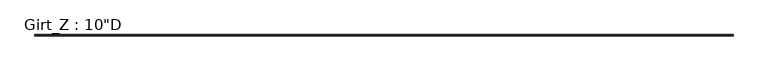
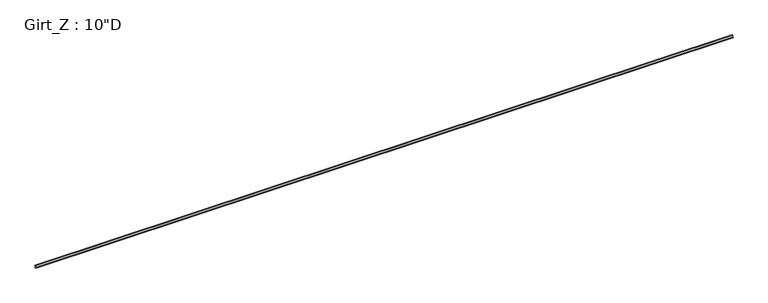
"""IFC4 building model written with IfcOpenShell, lengths in millimetres: beam geometry."""

from ifc_helpers import new_model, si_unit, point, frame, frame_2d, origin, place, context, project, spatial, polyline, circle_curve, trimmed, segment, composite_curve, outline, extrude, source, transform, mapped, element, save


def beam_a0c63cd6(model_context):
    return source(origin(), model_context, "Body", "SweptSolid", [
        extrude(outline(composite_curve([segment(polyline([(77.9859375, 127.0), (90.2310415, 112.4068534), (88.1028742, 110.621109), (76.6904765, 124.221875), (3.3005807, 124.221875)]), True, "CONTINUOUS"), segment(trimmed(circle_curve(frame_2d((3.3741066, 122.2381931)), 1.9850441), [point((3.3005807, 124.221875))], [point((1.3890625, 122.2381931))], True, "CARTESIAN"), True, "CONTINUOUS"), segment(polyline([(1.3890625, 122.2381931), (1.3890625, -127.0), (-84.3359375, -127.0), (-96.5810415, -112.4068534), (-94.4528742, -110.621109), (-83.0404765, -124.221875), (-3.2694106, -124.221875)]), True, "CONTINUOUS"), segment(trimmed(circle_curve(frame_2d((-3.3748024, -122.2389339)), 1.9857399), [point((-3.2694106, -124.221875))], [point((-1.3890625, -122.2389339))], True, "CARTESIAN"), True, "CONTINUOUS"), segment(polyline([(-1.3890625, -122.2389339), (-1.3890625, 122.2375)]), True, "CONTINUOUS"), segment(trimmed(circle_curve(frame_2d((3.3734375, 122.2375)), 4.7625), [point((-1.3890625, 122.2375))], [point((3.3734375, 127.0))], False, "CARTESIAN"), True, "CONTINUOUS"), segment(polyline([(3.3734375, 127.0), (77.9859375, 127.0)]), True, "CONTINUOUS")], self_intersect=False)), frame((-44056.3, 0.0, 0.0), z_axis=(1.0, 0.0, 0.0), x_axis=(0.0, 1.0, 0.0)), (0.0, 0.0, 1.0), 88112.6),
    ])


if __name__ == "__main__":
    model = new_model("IFC4")
    model_context = context("Model", 3, world=origin())
    ifc_project = project(units=[si_unit("LENGTHUNIT", "METRE", prefix="MILLI")], contexts=[model_context])
    site = spatial("IfcSite", under=ifc_project)
    building = spatial("IfcBuilding", under=site)
    placement = place(None, origin())
    beam_shape = beam_a0c63cd6(model_context)
    element("IfcBeam", 1, ObjectType="Girt_Z : 10\"D", at=placement, inside=building, context=model_context, shape_type="MappedRepresentation", body=[
        mapped(beam_shape, transform((0.0, 0.0, 0.0), x_axis=(1.0, 0.0, 0.0), y_axis=(0.0, 1.0, 0.0), z_axis=(0.0, 0.0, 1.0))),
    ])
    save(model, "model.ifc")

# Revit data of these elements
# Type "Girt_Z : 10\"D"
#   half leg = 0' - 1 11/16"
#   Web_Thickness = 0' - 0 7/64"
#   Length [instance default] = 10' - 0"
#   Leg_2 = 0' - 3 3/8"
#   Leg_1 = 0' - 3 1/8"
#   Height = 0' - 10"
#   Structural Material [instance default] = none
